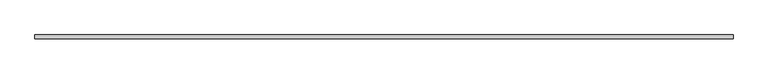
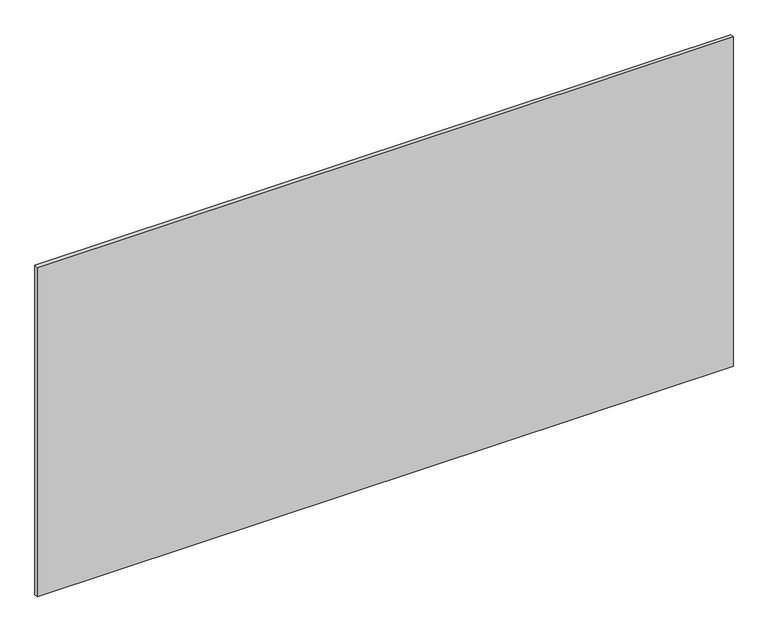
"""IFC4 building model written with IfcOpenShell, lengths in millimetres: proxy geometry, Inner panel:Inner panel:1:Inner panel:1 : Inner panel:Inner panel:300324:300043:Inner panel:1:Inner panel:1 : Inner panel:Inner panel:300324:300043 : Inner panel:Inner panel:1:Inner panel:1 : Inner panel:Inner panel:300324:300043:27 : Inner panel:Inner panel:1:Inner panel:1 : Inner panel:Inner panel:300324:300043:Inner panel:1:Inner panel:1 : Inner panel:Inner panel:300324:300043 : Inner panel:Inner panel:1:Inner panel:1 : Inner panel:Inner panel:300324:300043:300031."""

from ifc_helpers import new_model, si_unit, frame, origin, place, context, project, spatial, polyline, outline, extrude, source, transform, mapped, element, save


def generic_models_a279774f(model_context):
    return source(origin(), model_context, "Body", "SweptSolid", [
        extrude(outline(polyline([(593738.0867239, -579000.6913841), (596176.4867239, -579000.6913841), (596176.4867239, -579013.3913841), (593738.0867239, -579013.3913841), (593738.0867239, -579000.6913841)])), frame((0.0, 0.0, 1270.0), z_axis=(0.0, 0.0, 1.0), x_axis=(1.0, 0.0, 0.0)), (0.0, 0.0, 1.0), 1219.2),
    ])


if __name__ == "__main__":
    model = new_model("IFC4")
    model_context = context("Model", 3, world=origin())
    ifc_project = project(units=[si_unit("LENGTHUNIT", "METRE", prefix="MILLI")], contexts=[model_context])
    site = spatial("IfcSite", under=ifc_project)
    building = spatial("IfcBuilding", under=site)
    placement = place(None, origin())
    generic_models_shape = generic_models_a279774f(model_context)
    element("IfcBuildingElementProxy", 1, Name="Inner panel:Inner panel:1:Inner panel:1 : Inner panel:Inner panel:300324:300043:Inner panel:1:Inner panel:1 : Inner panel:Inner panel:300324:300043 : Inner panel:Inner panel:1:Inner panel:1 : Inner panel:Inner panel:300324:300043:27 : Inner panel:Inner panel:1:Inner panel:1 : Inner panel:Inner panel:300324:300043:Inner panel:1:Inner panel:1 : Inner panel:Inner panel:300324:300043 : Inner panel:Inner panel:1:Inner panel:1 : Inner panel:Inner panel:300324:300043:300031", ObjectType="Inner panel:Inner panel:1:Inner panel:1 : Inner panel:Inner panel:300324:300043:Inner panel:1:Inner panel:1 : Inner panel:Inner panel:300324:300043 : Inner panel:Inner panel:1:Inner panel:1 : Inner panel:Inner panel:300324:300043:27 : Inner panel:Inner panel:1:Inner panel:1 : Inner panel:Inner panel:300324:300043:Inner panel:1:Inner panel:1 : Inner panel:Inner panel:300324:300043 : Inner panel:Inner panel:1:Inner panel:1 : Inner panel:Inner panel:300324:300043:300031", at=placement, inside=building, context=model_context, shape_type="MappedRepresentation", body=[
        mapped(generic_models_shape, transform((0.0, 0.0, 0.0), x_axis=(1.0, 0.0, 0.0), y_axis=(0.0, 1.0, 0.0), z_axis=(0.0, 0.0, 1.0))),
    ])
    save(model, "model.ifc")

# Revit data of these elements
# Type "Inner panel:Inner panel:1:Inner panel:1 : Inner panel:Inner panel:300324:300043:Inner panel:1:Inner panel:1 : Inner panel:Inner panel:300324:300043 : Inner panel:Inner panel:1:Inner panel:1 : Inner panel:Inner panel:300324:300043:27 : Inner panel:Inner panel:1:Inner panel:1 : Inner panel:Inner panel:300324:300043:Inner panel:1:Inner panel:1 : Inner panel:Inner panel:300324:300043 : Inner panel:Inner panel:1:Inner panel:1 : Inner panel:Inner panel:300324:300043:300031"
#   NameOverride = "Inner panel:Inner panel:1:Inner panel:1 : Inner panel:Inner panel:300324:300043:Inner panel:1:Inner panel:1 : Inner panel:Inner panel:300324:300043 : Inner panel:Inner panel:1:Inner panel:1 : Inner panel:Inner panel:300324:300043:300031"
#   ObjectTypeOverride = "Inner panel:1:Inner panel:1 : Inner panel:Inner panel:300324:300043 : Inner panel:Inner panel:1:Inner panel:1 : Inner panel:Inner panel:300324:300043"
#   Reference = "Inner panel"
#   Tag = "300031"
# Element 1 (IfcBuildingElementProxy, "Inner panel:Inner panel:1:Inner panel:1 : Inner panel:Inner panel:300324:300043:Inner panel:1:Inner panel:1 : Inner panel:Inner panel:300324:300043 : Inner panel:Inner panel:1:Inner panel:1 : Inner panel:Inner panel:300324:300043:27 : Inner panel:Inner panel:1:Inner panel:1 : Inner panel:Inner panel:300324:300043:Inner panel:1:Inner panel:1 : Inner panel:Inner panel:300324:300043 : Inner panel:Inner panel:1:Inner panel:1 : Inner panel:Inner panel:300324:300043:300031")
#   Materials on its faces: "1/2\" EXTERIOR GRADE FIRE RETARDANT CDX PLYWOOD"
# Materials
#   "1/2\" EXTERIOR GRADE FIRE RETARDANT CDX PLYWOOD": class "Unassigned", colour RGB 196 177 123, transparency 0, Cost = 0
